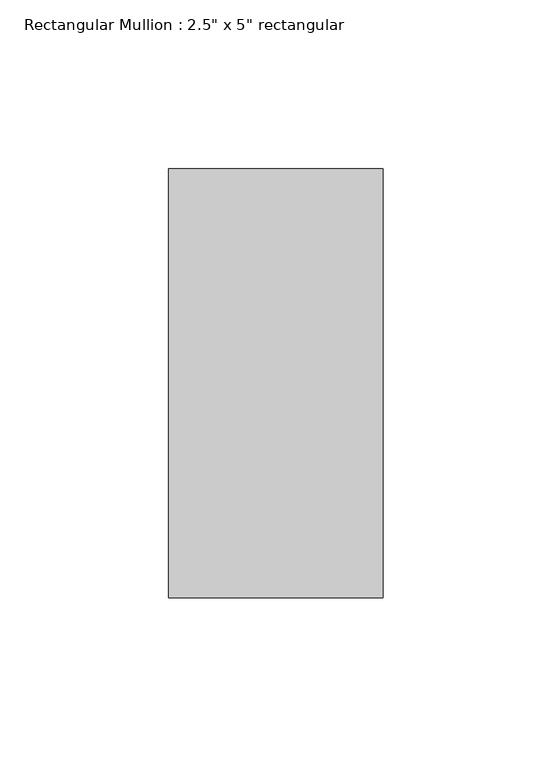
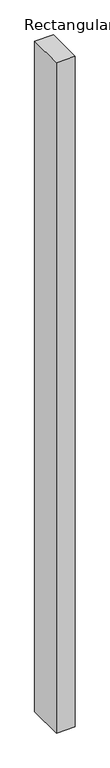
"""IFC4 building model written with IfcOpenShell, lengths in millimetres: member geometry."""

import ifcopenshell
import ifcopenshell.guid

model = None  # the IFC model being written
_history = None  # IfcOwnerHistory: only IFC2X3 demands one
_inside = {}  # id of a spatial element -> (the spatial element, [elements in it])
_under = {}  # id of a project, library or spatial element -> (it, [spatial elements below it])
_declared = {}  # id of a project -> (the project, [libraries it declares])
_typed = {}  # id of a type object -> (the type object, [elements of that type])
_made_of = {}  # id of a material, layer set ... -> (it, [elements and type objects made of it])


def new_model(schema):
    """Start an empty IFC model of exactly this schema.

    Asked for "IFC4X3", IfcOpenShell would pick the latest addendum, in which some entities
    have other attributes; the version numbers below select the first issue.
    IFC2X3 requires an IfcOwnerHistory on every rooted entity: one is made here for all.
    """
    global model, _history
    if schema == "IFC4X3":
        model = ifcopenshell.file(schema_version=(4, 3, 0, 0))
    else:
        model = ifcopenshell.file(schema=schema)
    _inside.clear()
    _under.clear()
    _declared.clear()
    _typed.clear()
    _made_of.clear()
    _history = None
    if model.schema == "IFC2X3":
        org = make("IfcOrganization", Name="unknown")
        user = make(
            "IfcPersonAndOrganization",
            ThePerson=make("IfcPerson", FamilyName="unknown"),
            TheOrganization=org,
        )
        app = make(
            "IfcApplication",
            ApplicationDeveloper=org,
            Version="unknown",
            ApplicationFullName="unknown",
            ApplicationIdentifier="unknown",
        )
        _history = make(
            "IfcOwnerHistory",
            OwningUser=user,
            OwningApplication=app,
            ChangeAction="ADDED",
            CreationDate=0,
        )
    return model


def make(cls, **values):
    """One entity of the class cls with the attributes given. An attribute that is None is left unset."""
    return model.create_entity(
        cls, **{name: value for name, value in values.items() if value is not None}
    )


def rooted(cls, **values):
    """An entity with a GlobalId (a new one), such as an element, a storey or a relation."""
    return make(cls, GlobalId=ifcopenshell.guid.new(), OwnerHistory=_history, **values)


def si_unit(unit_type, name, prefix=None):
    """IfcSIUnit, for example si_unit("LENGTHUNIT", "METRE", prefix="MILLI")."""
    return make("IfcSIUnit", UnitType=unit_type, Prefix=prefix, Name=name)


def assignment(units):
    """IfcUnitAssignment: the units of a project."""
    return None if units is None else make("IfcUnitAssignment", Units=units)


def point(xyz):
    """IfcCartesianPoint."""
    return None if xyz is None else make("IfcCartesianPoint", Coordinates=xyz)


def direction(xyz):
    """IfcDirection."""
    return None if xyz is None else make("IfcDirection", DirectionRatios=xyz)


def frame(location, z_axis=None, x_axis=None):
    """IfcAxis2Placement3D, a coordinate frame: its origin and axes. An axis left out is left unset."""
    return make(
        "IfcAxis2Placement3D",
        Location=point(location),
        Axis=direction(z_axis),
        RefDirection=direction(x_axis),
    )


def origin():
    """The frame at (0, 0, 0) with its axes left unset."""
    return frame((0.0, 0.0, 0.0))


def place(relative_to, where):
    """IfcLocalPlacement: puts the frame where relative to a parent placement (None: the world)."""
    return make(
        "IfcLocalPlacement", PlacementRelTo=relative_to, RelativePlacement=where
    )


def context(
    kind, dimensions, precision=None, world=None, true_north=None, identifier=None
):
    """IfcGeometricRepresentationContext, for example the 3D "Model" context."""
    return make(
        "IfcGeometricRepresentationContext",
        ContextIdentifier=identifier,
        ContextType=kind,
        CoordinateSpaceDimension=dimensions,
        Precision=precision,
        WorldCoordinateSystem=world,
        TrueNorth=true_north,
    )


def project(units=None, contexts=None):
    """IfcProject with its units and contexts."""
    return rooted(
        "IfcProject",
        Name="project",
        RepresentationContexts=contexts,
        UnitsInContext=assignment(units),
    )


def spatial(cls, under=None, at=None, **own):
    """A site, building, storey or space (cls), placed at a placement, below another one or the project."""
    s = rooted(cls, ObjectPlacement=at, **own)
    if under is not None:
        _under.setdefault(under.id(), (under, []))[1].append(s)
    return s


def polyline(points):
    """IfcPolyline through the points."""
    return make("IfcPolyline", Points=[point(p) for p in points])


def outline(outer, holes=None, kind="AREA"):
    """IfcArbitraryClosedProfileDef: a profile drawn as a closed curve; with holes, ...WithVoids."""
    if holes is None:
        return make("IfcArbitraryClosedProfileDef", ProfileType=kind, OuterCurve=outer)
    return make(
        "IfcArbitraryProfileDefWithVoids",
        ProfileType=kind,
        OuterCurve=outer,
        InnerCurves=holes,
    )


def extrude(swept, where, along, depth):
    """IfcExtrudedAreaSolid: the profile swept, set in the frame where, extruded along a direction by depth."""
    return make(
        "IfcExtrudedAreaSolid",
        SweptArea=swept,
        Position=where,
        ExtrudedDirection=direction(along),
        Depth=depth,
    )


def shape(context_of_items, identifier, shape_type, items):
    """IfcShapeRepresentation: the items that make up one representation, for example the "Body"."""
    return make(
        "IfcShapeRepresentation",
        ContextOfItems=context_of_items,
        RepresentationIdentifier=identifier,
        RepresentationType=shape_type,
        Items=items,
    )


def source(mapping_origin, context_of_items, identifier, shape_type, items):
    """IfcRepresentationMap: a shape defined once, which mapped items show again and again."""
    return make(
        "IfcRepresentationMap",
        MappingOrigin=mapping_origin,
        MappedRepresentation=shape(context_of_items, identifier, shape_type, items),
    )


def transform(
    local_origin,
    x_axis=None,
    y_axis=None,
    z_axis=None,
    scale=None,
    scale2=None,
    scale3=None,
    uniform=True,
):
    """IfcCartesianTransformationOperator3D, or its non-uniform kind. x_axis, y_axis, z_axis: its Axis1, 2, 3."""
    if uniform:
        return make(
            "IfcCartesianTransformationOperator3D",
            Axis1=direction(x_axis),
            Axis2=direction(y_axis),
            LocalOrigin=point(local_origin),
            Scale=scale,
            Axis3=direction(z_axis),
        )
    return make(
        "IfcCartesianTransformationOperator3DnonUniform",
        Axis1=direction(x_axis),
        Axis2=direction(y_axis),
        LocalOrigin=point(local_origin),
        Scale=scale,
        Axis3=direction(z_axis),
        Scale2=scale2,
        Scale3=scale3,
    )


def mapped(mapping_source, mapping_target):
    """IfcMappedItem: shows the shape of a source again, moved by a transform."""
    return make(
        "IfcMappedItem", MappingSource=mapping_source, MappingTarget=mapping_target
    )


def made_of(thing, what):
    """Note that an element or type object is made of a material, layer set ...; save() writes the relation."""
    if what is not None:
        _made_of.setdefault(what.id(), (what, []))[1].append(thing)
    return thing


def element(
    cls,
    number,
    at=None,
    inside=None,
    cuts=None,
    type_object=None,
    material=None,
    context=None,
    identifier="Body",
    shape_type=None,
    held_by="IfcProductDefinitionShape",
    body=None,
    shapes=None,
    **own,
):
    """One element of the class cls, such as IfcWall. Its Tag is "e" and its number.

    at: its placement. inside: the storey or other place that contains it. cuts: it is an
    opening in that element (IfcRelVoidsElement). A single representation is given by context,
    identifier, shape_type and body (its items); several are given by shapes. held_by: the class
    of the entity that holds the representations. save() writes the other relations.
    """
    e = rooted(cls, Tag="e%d" % number, ObjectPlacement=at, **own)
    if body is not None:
        shapes = [shape(context, identifier, shape_type, body)]
    if shapes is not None:
        e.Representation = make(held_by, Representations=shapes)
    if inside is not None:
        _inside.setdefault(inside.id(), (inside, []))[1].append(e)
    if cuts is not None:
        rooted(
            "IfcRelVoidsElement", RelatingBuildingElement=cuts, RelatedOpeningElement=e
        )
    if type_object is not None:
        _typed.setdefault(type_object.id(), (type_object, []))[1].append(e)
    return made_of(e, material)


def aggregate(whole, parts):
    """IfcRelAggregates: a whole, such as a stair, and the parts it consists of."""
    return rooted("IfcRelAggregates", RelatingObject=whole, RelatedObjects=parts)


def save(model, path):
    """Write the relations noted so far, then the file.

    IfcRelAggregates (storeys below a building ...), IfcRelContainedInSpatialStructure (elements
    in a storey), IfcRelDefinesByType, IfcRelAssociatesMaterial and IfcRelDeclares: one each for
    every whole, place, type object, material and project.
    """
    for whole, parts in _under.values():
        aggregate(whole, parts)
    for where, things in _inside.values():
        rooted(
            "IfcRelContainedInSpatialStructure",
            RelatedElements=things,
            RelatingStructure=where,
        )
    for kind, things in _typed.values():
        rooted("IfcRelDefinesByType", RelatedObjects=things, RelatingType=kind)
    for what, things in _made_of.values():
        rooted("IfcRelAssociatesMaterial", RelatedObjects=things, RelatingMaterial=what)
    for by, libraries in _declared.values():
        rooted("IfcRelDeclares", RelatingContext=by, RelatedDefinitions=libraries)
    model.write(path)


def member_92b946c3(model_context):
    return source(origin(), model_context, "Body", "SweptSolid", [
        extrude(outline(polyline([(31.75, 63.5), (31.75, -63.5), (-31.75, -63.5), (-31.75, 63.5), (31.75, 63.5)])), frame((0.0, 0.0, -2406.65), z_axis=(0.0, 0.0, 1.0), x_axis=(1.0, 0.0, 0.0)), (0.0, 0.0, 1.0), 2406.65),
    ])


if __name__ == "__main__":
    model = new_model("IFC4")
    model_context = context("Model", 3, world=origin())
    ifc_project = project(units=[si_unit("LENGTHUNIT", "METRE", prefix="MILLI")], contexts=[model_context])
    site = spatial("IfcSite", under=ifc_project)
    building = spatial("IfcBuilding", under=site)
    placement = place(None, origin())
    member_shape = member_92b946c3(model_context)
    element("IfcMember", 1, ObjectType="Rectangular Mullion : 2.5\" x 5\" rectangular", at=placement, inside=building, context=model_context, shape_type="MappedRepresentation", body=[
        mapped(member_shape, transform((0.0, 0.0, 0.0), x_axis=(1.0, 0.0, 0.0), y_axis=(0.0, 1.0, 0.0), z_axis=(0.0, 0.0, 1.0))),
    ])
    save(model, "model.ifc")

# Revit data of these elements
# Type "Rectangular Mullion : 2.5\" x 5\" rectangular"
#   built-in parameter 1007304 = 0.416667 (stored number, unit not read)
#   built-in parameter 1007301 = 0.104167 (stored number, unit not read)
#   built-in parameter 1007300 = 0.104167 (stored number, unit not read)
# Element 1 (IfcMember, "Rectangular Mullion : 2.5\" x 5\" rectangular")
#   Materials on its faces: "Aluminum"
# Materials
#   "Aluminum": class "Metal", colour RGB 247 247 247, transparency 0, Description = "Aluminum 6061", Cost = 0
